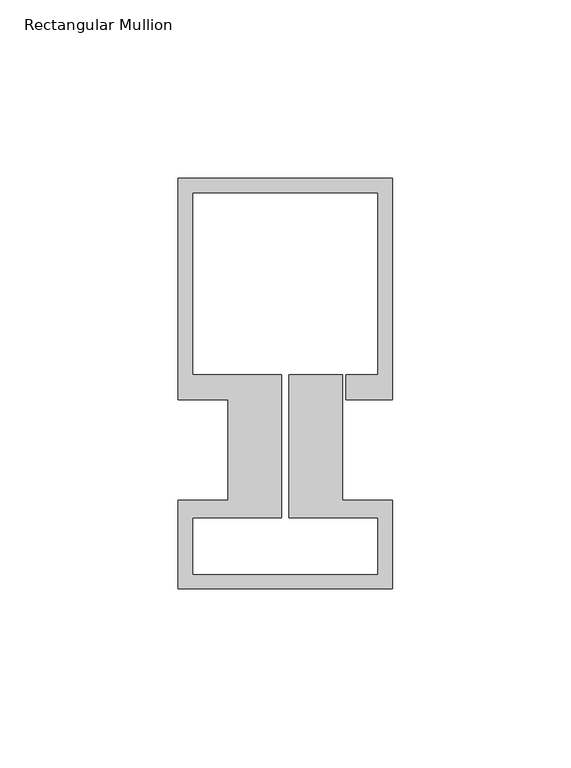
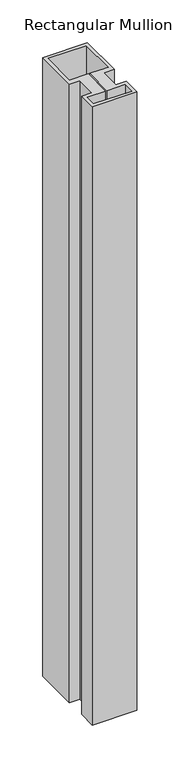
"""IFC4 building model written with IfcOpenShell, lengths in millimetres: member geometry, Rectangular Mullion : Schueco_FWS-60-HI_Tran_CovCap-20mm_Tran-55mm."""

from ifc_helpers import new_model, si_unit, frame, origin, place, context, project, spatial, polyline, outline, extrude, source, transform, mapped, element, save


def rectangular_mullion_83b4649c(model_context):
    return source(origin(), model_context, "Body", "SweptSolid", [
        extrude(outline(polyline([(-60.0, 90.0), (0.0, 90.0), (0.0, 28.0), (-13.0, 28.0), (-13.0, 35.0), (-4.0, 35.0), (-4.0, 86.0), (-56.0, 86.0), (-56.0, 35.0), (-31.0, 35.0), (-31.0, -5.0), (-56.0, -5.0), (-56.0, -21.0), (-4.0, -21.0), (-4.0, -5.0), (-29.0, -5.0), (-29.0, 35.0), (-14.0, 35.0), (-14.0, -0.1), (0.0, -0.1), (0.0, -25.0), (-60.0, -25.0), (-60.0, -0.1), (-46.0, -0.1), (-46.0, 28.0), (-60.0, 28.0), (-60.0, 90.0)])), frame((0.0, 0.0, -880.0), z_axis=(0.0, 0.0, 1.0), x_axis=(1.0, 0.0, 0.0)), (0.0, 0.0, 1.0), 880.0),
    ])


if __name__ == "__main__":
    model = new_model("IFC4")
    model_context = context("Model", 3, world=origin())
    ifc_project = project(units=[si_unit("LENGTHUNIT", "METRE", prefix="MILLI")], contexts=[model_context])
    site = spatial("IfcSite", under=ifc_project)
    building = spatial("IfcBuilding", under=site)
    placement = place(None, origin())
    rectangular_mullion_shape = rectangular_mullion_83b4649c(model_context)
    element("IfcMember", 1, ObjectType="Rectangular Mullion : Schueco_FWS-60-HI_Tran_CovCap-20mm_Tran-55mm", at=placement, inside=building, context=model_context, shape_type="MappedRepresentation", body=[
        mapped(rectangular_mullion_shape, transform((0.0, 0.0, 0.0), x_axis=(1.0, 0.0, 0.0), y_axis=(0.0, 1.0, 0.0), z_axis=(0.0, 0.0, 1.0))),
    ])
    save(model, "model.ifc")

# Revit data of these elements
# Type "Rectangular Mullion : Schueco_FWS-60-HI_Tran_CovCap-20mm_Tran-55mm"
#   Model = "FWS 60.HI"
#   Manufacturer = "Schueco International KG"
#   Type Comments = "Transom"
#   Schueco thermal insulation standard = "Highly thermally insulated"
#   Burglar resistance = "RC 3"
#   Thermal insulation = "to 0.90 W/(m²K)"
#   built-in parameter 1007322 = 0.377297 (stored number, unit not read)
#   built-in parameter 1007321 = 0.0524934 (stored number, unit not read)
#   built-in parameter 1007320 = 0.0524934 (stored number, unit not read)
# Element 1 (IfcMember, "Rectangular Mullion : Schueco_FWS-60-HI_Tran_CovCap-20mm_Tran-55mm")
#   Materials on its faces: "Alu"
# Materials
#   "Alu": class "Glas", colour RGB 140 140 140, transparency 0
